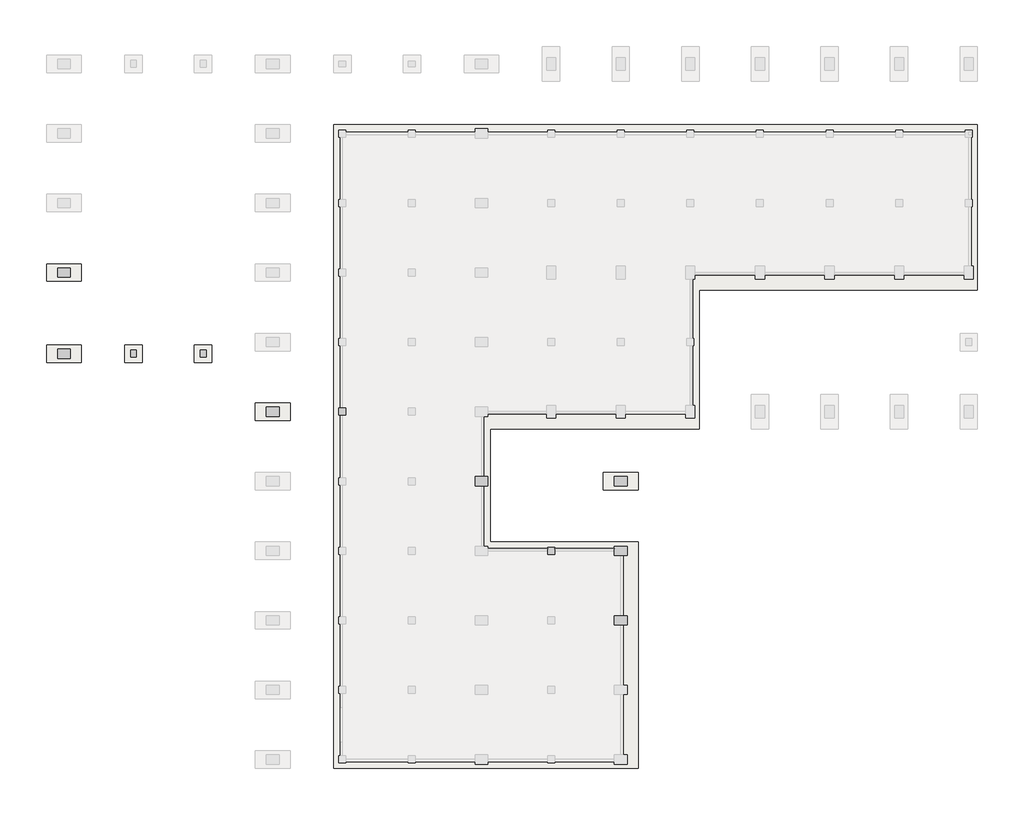
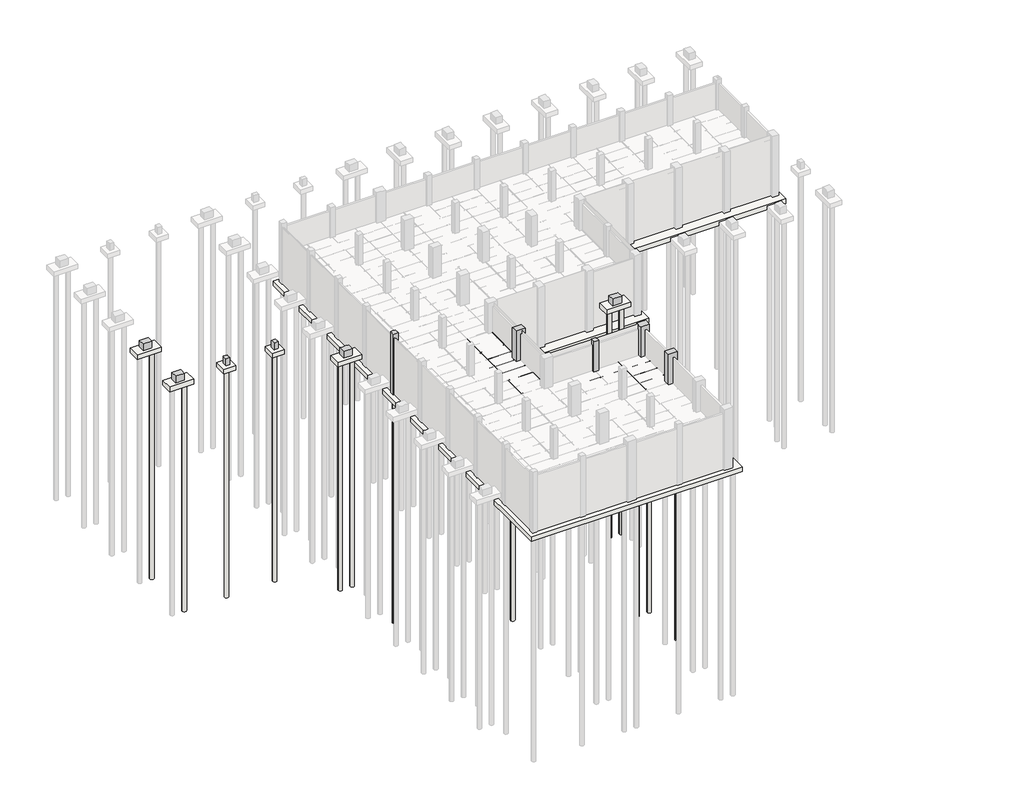
# Not in any storey, part 6 of 16: 20 slabs, 16 beams, 11 columns.
# Revit data of these elements (continued)
# Elements 1, 3, 4, 5, 6, 7, 11, 12, 15, 16 (IfcBeam, "Steel Framing_C_KS : H_SB_AR_S02_C-150x75x6.5x10_J1") (continued)
#   Materials on its faces: "Steel, 45-345"
# Elements 2, 10, 14 (IfcBeam, "Steel Framing_H_KS : H_SB_AR_S02_H-400x200x8x13_BSB1")
#   Structural Material = Steel, 45-345
#   Phase Created = New Construction
#   Materials on its faces: "Steel, 45-345"
# Element 8 (IfcBeam, "Steel Framing_H_KS : H_SB_AR_S02_H-400x200x8x13_BSG1")
#   Structural Material = Steel, 45-345
#   Phase Created = New Construction
#   Materials on its faces: "Steel, 45-345"
# Elements 9, 13 (IfcBeam, "Steel Framing_H_KS : H_SB_AR_S02_H-400x200x8x13_BSG2")
#   Structural Material = Steel, 45-345
#   Phase Created = New Construction
#   Materials on its faces: "Steel, 45-345"
# Elements 17, 18, 19, 20, 21, 22, 23 (IfcColumn, "RC_Column_Rectangular : H_SC_AR_S15_UG PED_Bit_800x1100_PD1")
#   Comments = ""
#   hec_material3 = none
#   hec_material2 = none
#   hec_material1 = none
#   Structural Material = 00_Concrete_Reinf. Conc.
#   Phase Created = New Construction
#   Materials on its faces: "00_Concrete_Reinf. Conc."
# Elements 24, 25 (IfcColumn, "RC_Column_Rectangular : H_SC_AR_S15_UG PED_Bit_600x600_BC1")
#   Comments = ""
#   hec_material3 = none
#   hec_material2 = none
#   hec_material1 = none
#   Structural Material = 00_Concrete_Reinf. Conc.
#   Phase Created = New Construction
#   Materials on its faces: "00_Concrete_Reinf. Conc."
# Elements 26, 27 (IfcColumn, "RC_Column_Rectangular : H_SC_AR_S15_UG PED_Bit_500x600_PD2")
#   Comments = ""
#   hec_material3 = none
#   hec_material2 = none
#   hec_material1 = none
#   Structural Material = 00_Concrete_Reinf. Conc.
#   Phase Created = New Construction
#   Materials on its faces: "00_Concrete_Reinf. Conc."
# Element 28 (IfcSlab, "H_SF_AR_S18_MAT_Bitumen_T600_MF1")
#   Comments = ""
#   Height Offset From Level = 0 mm
#   built-in parameter 1001954 = 1
#   Phase Created = New Construction
#   Materials on its faces: "00_Concrete_Reinf. Conc."
# Elements 29, 30, 31, 32 (IfcSlab, "Foundation Rectangular (Non-Pile) : H_SF_AR_S18_Shallow Fdn_Bitumen_1500x3000xT600_F1")
#   Comments = ""
#   Structural Material = 00_Concrete_Reinf. Conc.
#   Phase Created = New Construction
#   Materials on its faces: "00_Concrete_Reinf. Conc."
# Elements 33, 34 (IfcSlab, "Foundation Rectangular (Non-Pile) : H_SF_AR_S18_Shallow Fdn_Bitumen_1500x1500xT600_F2")
#   Comments = ""
#   Structural Material = 00_Concrete_Reinf. Conc.
#   Phase Created = New Construction
#   Materials on its faces: "00_Concrete_Reinf. Conc."
# Elements 35, 36, 37, 38, 39, 40, 41, 42 (IfcSlab, "PILE : H_SF_AR_S19_PHC Pile_Pre-boring_D500_L30")
#   Structural Material = Concrete, Precast
#   Phase Created = New Construction
#   Materials on its faces: "Concrete, Precast"
# Elements 43, 44, 45, 46, 47 (IfcSlab, "PILE : H_SF_AR_S19_PHC Pile_Pre-boring_D500_L30")
#   Structural Material = none
#   Phase Created = New Construction
# Materials
#   "Steel, 45-345": class "Metal", colour RGB 189 187 185, transparency 0, Description = "Steel 345 MPa", Cost = 0
#   "00_Concrete_Reinf. Conc.": class "Concrete", colour RGB 176 176 176, transparency 0, Description = "Reinf. Conc.", Cost = 0, Image = Concrete.Cast-In-Place.Flat.Polished.Grey.jpg
#   "Concrete, Precast": class "Concrete", colour RGB 115 116 108, transparency 0, Description = "Precast concrete", Cost = 0
